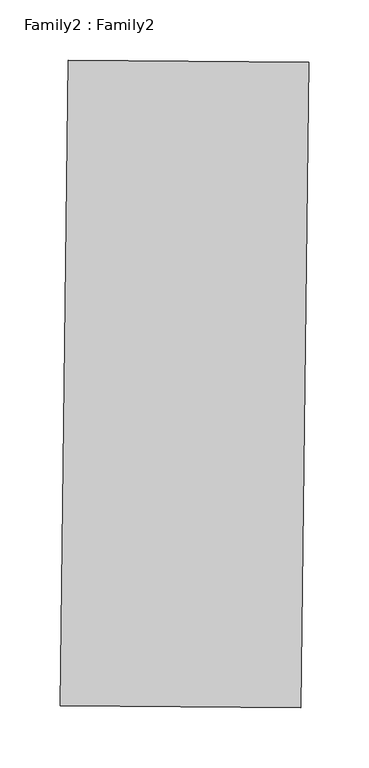
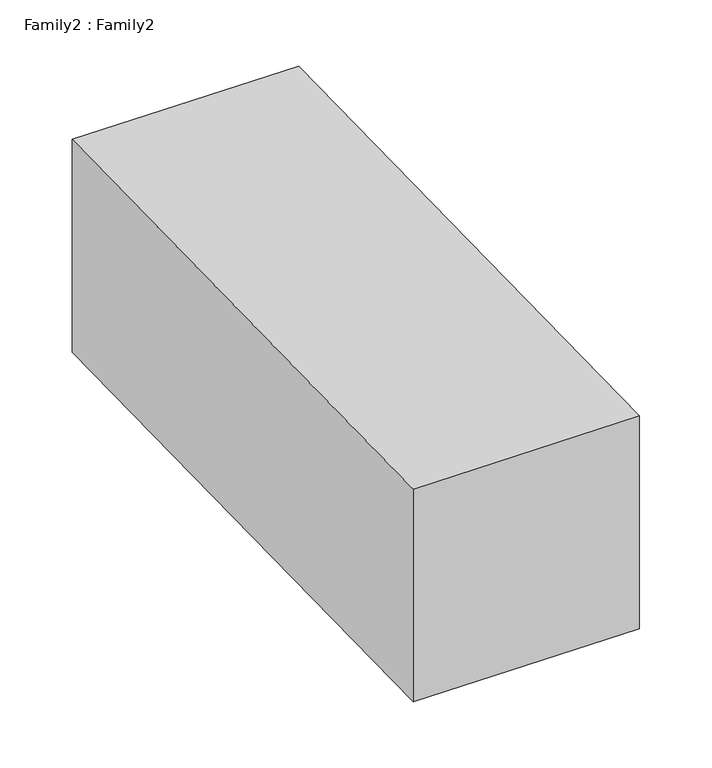
"""IFC4 building model written with IfcOpenShell, lengths in millimetres: proxy geometry, Family2 : Family2."""

import ifcopenshell
import ifcopenshell.guid

model = None  # the IFC model being written
_history = None  # IfcOwnerHistory: only IFC2X3 demands one
_inside = {}  # id of a spatial element -> (the spatial element, [elements in it])
_under = {}  # id of a project, library or spatial element -> (it, [spatial elements below it])
_declared = {}  # id of a project -> (the project, [libraries it declares])
_typed = {}  # id of a type object -> (the type object, [elements of that type])
_made_of = {}  # id of a material, layer set ... -> (it, [elements and type objects made of it])


def new_model(schema):
    """Start an empty IFC model of exactly this schema.

    Asked for "IFC4X3", IfcOpenShell would pick the latest addendum, in which some entities
    have other attributes; the version numbers below select the first issue.
    IFC2X3 requires an IfcOwnerHistory on every rooted entity: one is made here for all.
    """
    global model, _history
    if schema == "IFC4X3":
        model = ifcopenshell.file(schema_version=(4, 3, 0, 0))
    else:
        model = ifcopenshell.file(schema=schema)
    _inside.clear()
    _under.clear()
    _declared.clear()
    _typed.clear()
    _made_of.clear()
    _history = None
    if model.schema == "IFC2X3":
        org = make("IfcOrganization", Name="unknown")
        user = make(
            "IfcPersonAndOrganization",
            ThePerson=make("IfcPerson", FamilyName="unknown"),
            TheOrganization=org,
        )
        app = make(
            "IfcApplication",
            ApplicationDeveloper=org,
            Version="unknown",
            ApplicationFullName="unknown",
            ApplicationIdentifier="unknown",
        )
        _history = make(
            "IfcOwnerHistory",
            OwningUser=user,
            OwningApplication=app,
            ChangeAction="ADDED",
            CreationDate=0,
        )
    return model


def make(cls, **values):
    """One entity of the class cls with the attributes given. An attribute that is None is left unset."""
    return model.create_entity(
        cls, **{name: value for name, value in values.items() if value is not None}
    )


def rooted(cls, **values):
    """An entity with a GlobalId (a new one), such as an element, a storey or a relation."""
    return make(cls, GlobalId=ifcopenshell.guid.new(), OwnerHistory=_history, **values)


def si_unit(unit_type, name, prefix=None):
    """IfcSIUnit, for example si_unit("LENGTHUNIT", "METRE", prefix="MILLI")."""
    return make("IfcSIUnit", UnitType=unit_type, Prefix=prefix, Name=name)


def assignment(units):
    """IfcUnitAssignment: the units of a project."""
    return None if units is None else make("IfcUnitAssignment", Units=units)


def point(xyz):
    """IfcCartesianPoint."""
    return None if xyz is None else make("IfcCartesianPoint", Coordinates=xyz)


def direction(xyz):
    """IfcDirection."""
    return None if xyz is None else make("IfcDirection", DirectionRatios=xyz)


def frame(location, z_axis=None, x_axis=None):
    """IfcAxis2Placement3D, a coordinate frame: its origin and axes. An axis left out is left unset."""
    return make(
        "IfcAxis2Placement3D",
        Location=point(location),
        Axis=direction(z_axis),
        RefDirection=direction(x_axis),
    )


def origin():
    """The frame at (0, 0, 0) with its axes left unset."""
    return frame((0.0, 0.0, 0.0))


def place(relative_to, where):
    """IfcLocalPlacement: puts the frame where relative to a parent placement (None: the world)."""
    return make(
        "IfcLocalPlacement", PlacementRelTo=relative_to, RelativePlacement=where
    )


def context(
    kind, dimensions, precision=None, world=None, true_north=None, identifier=None
):
    """IfcGeometricRepresentationContext, for example the 3D "Model" context."""
    return make(
        "IfcGeometricRepresentationContext",
        ContextIdentifier=identifier,
        ContextType=kind,
        CoordinateSpaceDimension=dimensions,
        Precision=precision,
        WorldCoordinateSystem=world,
        TrueNorth=true_north,
    )


def project(units=None, contexts=None):
    """IfcProject with its units and contexts."""
    return rooted(
        "IfcProject",
        Name="project",
        RepresentationContexts=contexts,
        UnitsInContext=assignment(units),
    )


def spatial(cls, under=None, at=None, **own):
    """A site, building, storey or space (cls), placed at a placement, below another one or the project."""
    s = rooted(cls, ObjectPlacement=at, **own)
    if under is not None:
        _under.setdefault(under.id(), (under, []))[1].append(s)
    return s


def faces_of(points, faces, orient=None, outer=None):
    """IfcFace entities. A face is a list of loops; a loop is a list of indices into points, from 0.

    orient and outer hold one flag for each loop. By default every Orientation is true, the
    first loop of a face is its IfcFaceOuterBound and the others are IfcFaceBound.
    """
    made = []
    for i, loops in enumerate(faces):
        bounds = []
        for j, loop in enumerate(loops):
            is_outer = j == 0 if outer is None else outer[i][j]
            bounds.append(
                make(
                    "IfcFaceOuterBound" if is_outer else "IfcFaceBound",
                    Bound=make("IfcPolyLoop", Polygon=[points[k] for k in loop]),
                    Orientation=True if orient is None else orient[i][j],
                )
            )
        made.append(make("IfcFace", Bounds=bounds))
    return made


def faceted_brep(points, faces, orient=None, outer=None, voids=None):
    """IfcFacetedBrep: a solid bounded by flat faces; with voids (closed shells), ...WithVoids."""
    shared = [point(p) for p in points]
    hull = make("IfcClosedShell", CfsFaces=faces_of(shared, faces, orient, outer))
    if voids is None:
        return make("IfcFacetedBrep", Outer=hull)
    return make(
        "IfcFacetedBrepWithVoids",
        Outer=hull,
        Voids=[
            make(cls, CfsFaces=faces_of(shared, fs, o, b)) for cls, fs, o, b in voids
        ],
    )


def shape(context_of_items, identifier, shape_type, items):
    """IfcShapeRepresentation: the items that make up one representation, for example the "Body"."""
    return make(
        "IfcShapeRepresentation",
        ContextOfItems=context_of_items,
        RepresentationIdentifier=identifier,
        RepresentationType=shape_type,
        Items=items,
    )


def source(mapping_origin, context_of_items, identifier, shape_type, items):
    """IfcRepresentationMap: a shape defined once, which mapped items show again and again."""
    return make(
        "IfcRepresentationMap",
        MappingOrigin=mapping_origin,
        MappedRepresentation=shape(context_of_items, identifier, shape_type, items),
    )


def transform(
    local_origin,
    x_axis=None,
    y_axis=None,
    z_axis=None,
    scale=None,
    scale2=None,
    scale3=None,
    uniform=True,
):
    """IfcCartesianTransformationOperator3D, or its non-uniform kind. x_axis, y_axis, z_axis: its Axis1, 2, 3."""
    if uniform:
        return make(
            "IfcCartesianTransformationOperator3D",
            Axis1=direction(x_axis),
            Axis2=direction(y_axis),
            LocalOrigin=point(local_origin),
            Scale=scale,
            Axis3=direction(z_axis),
        )
    return make(
        "IfcCartesianTransformationOperator3DnonUniform",
        Axis1=direction(x_axis),
        Axis2=direction(y_axis),
        LocalOrigin=point(local_origin),
        Scale=scale,
        Axis3=direction(z_axis),
        Scale2=scale2,
        Scale3=scale3,
    )


def mapped(mapping_source, mapping_target):
    """IfcMappedItem: shows the shape of a source again, moved by a transform."""
    return make(
        "IfcMappedItem", MappingSource=mapping_source, MappingTarget=mapping_target
    )


def made_of(thing, what):
    """Note that an element or type object is made of a material, layer set ...; save() writes the relation."""
    if what is not None:
        _made_of.setdefault(what.id(), (what, []))[1].append(thing)
    return thing


def element(
    cls,
    number,
    at=None,
    inside=None,
    cuts=None,
    type_object=None,
    material=None,
    context=None,
    identifier="Body",
    shape_type=None,
    held_by="IfcProductDefinitionShape",
    body=None,
    shapes=None,
    **own,
):
    """One element of the class cls, such as IfcWall. Its Tag is "e" and its number.

    at: its placement. inside: the storey or other place that contains it. cuts: it is an
    opening in that element (IfcRelVoidsElement). A single representation is given by context,
    identifier, shape_type and body (its items); several are given by shapes. held_by: the class
    of the entity that holds the representations. save() writes the other relations.
    """
    e = rooted(cls, Tag="e%d" % number, ObjectPlacement=at, **own)
    if body is not None:
        shapes = [shape(context, identifier, shape_type, body)]
    if shapes is not None:
        e.Representation = make(held_by, Representations=shapes)
    if inside is not None:
        _inside.setdefault(inside.id(), (inside, []))[1].append(e)
    if cuts is not None:
        rooted(
            "IfcRelVoidsElement", RelatingBuildingElement=cuts, RelatedOpeningElement=e
        )
    if type_object is not None:
        _typed.setdefault(type_object.id(), (type_object, []))[1].append(e)
    return made_of(e, material)


def aggregate(whole, parts):
    """IfcRelAggregates: a whole, such as a stair, and the parts it consists of."""
    return rooted("IfcRelAggregates", RelatingObject=whole, RelatedObjects=parts)


def save(model, path):
    """Write the relations noted so far, then the file.

    IfcRelAggregates (storeys below a building ...), IfcRelContainedInSpatialStructure (elements
    in a storey), IfcRelDefinesByType, IfcRelAssociatesMaterial and IfcRelDeclares: one each for
    every whole, place, type object, material and project.
    """
    for whole, parts in _under.values():
        aggregate(whole, parts)
    for where, things in _inside.values():
        rooted(
            "IfcRelContainedInSpatialStructure",
            RelatedElements=things,
            RelatingStructure=where,
        )
    for kind, things in _typed.values():
        rooted("IfcRelDefinesByType", RelatedObjects=things, RelatingType=kind)
    for what, things in _made_of.values():
        rooted("IfcRelAssociatesMaterial", RelatedObjects=things, RelatingMaterial=what)
    for by, libraries in _declared.values():
        rooted("IfcRelDeclares", RelatingContext=by, RelatedDefinitions=libraries)
    model.write(path)


def family2_family2_c4a0287a(model_context):
    return source(origin(), model_context, "Body", "Brep", [
        faceted_brep([(-3946.7533915, -6341.9967642, 1.0945136), (-3946.7533915, -6341.9967642, 201.0945136), (-3940.089403, -5805.6033584, 202.060409), (-3940.089403, -5805.6033584, 2.060409), (-3746.7622015, -6343.8739769, 201.0945136), (-3740.098213, -5807.480571, 202.060409), (-3746.7622015, -6343.8739769, 1.0945136), (-3740.098213, -5807.480571, 2.060409)], [[[0, 1, 2, 3]], [[1, 4, 5, 2]], [[4, 6, 7, 5]], [[6, 0, 3, 7]], [[3, 2, 5, 7]], [[0, 6, 4, 1]]]),
    ])


if __name__ == "__main__":
    model = new_model("IFC4")
    model_context = context("Model", 3, world=origin())
    ifc_project = project(units=[si_unit("LENGTHUNIT", "METRE", prefix="MILLI")], contexts=[model_context])
    site = spatial("IfcSite", under=ifc_project)
    building = spatial("IfcBuilding", under=site)
    placement = place(None, origin())
    family2_family2_shape = family2_family2_c4a0287a(model_context)
    element("IfcBuildingElementProxy", 1, Name="Family2 : Family2", ObjectType="Family2 : Family2", at=placement, inside=building, context=model_context, shape_type="MappedRepresentation", body=[
        mapped(family2_family2_shape, transform((0.0, 0.0, 0.0), x_axis=(1.0, 0.0, 0.0), y_axis=(0.0, 1.0, 0.0), z_axis=(0.0, 0.0, 1.0))),
    ])
    save(model, "model.ifc")

# Revit data of these elements
# Type "Family2 : Family2"
#   Default Elevation = 0
